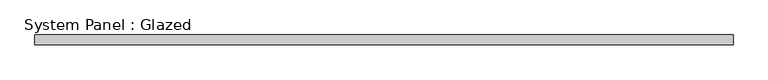
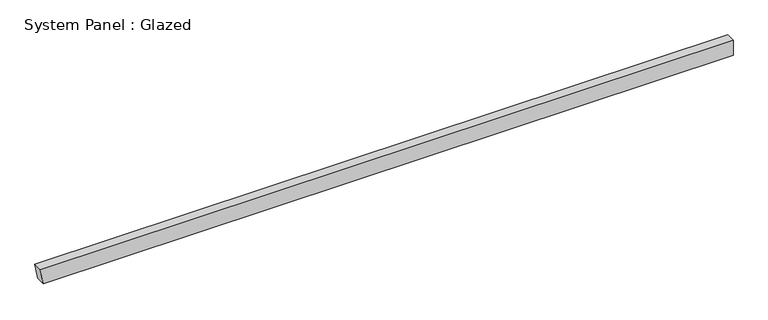
"""IFC4 building model written with IfcOpenShell, lengths in millimetres: plate geometry, System Panel : Glazed."""

from ifc_helpers import new_model, si_unit, frame, origin, place, context, project, spatial, polyline, outline, extrude, source, transform, mapped, element, save


def system_panel_glazed_0a43eb3e(model_context):
    return source(origin(), model_context, "Body", "SweptSolid", [
        extrude(outline(polyline([(0.0, -907.0374994), (0.0, 914.4000002), (41.9143134, 914.4000002), (41.9143134, -914.4000002), (0.0, -907.0374994)])), frame((0.0, -44.45, 0.0), z_axis=(0.0, 1.0, 0.0), x_axis=(0.0, 0.0, 1.0)), (0.0, 0.0, 1.0), 25.4),
    ])


if __name__ == "__main__":
    model = new_model("IFC4")
    model_context = context("Model", 3, world=origin())
    ifc_project = project(units=[si_unit("LENGTHUNIT", "METRE", prefix="MILLI")], contexts=[model_context])
    site = spatial("IfcSite", under=ifc_project)
    building = spatial("IfcBuilding", under=site)
    placement = place(None, origin())
    system_panel_glazed_shape = system_panel_glazed_0a43eb3e(model_context)
    element("IfcPlate", 1, ObjectType="System Panel : Glazed", at=placement, inside=building, context=model_context, shape_type="MappedRepresentation", body=[
        mapped(system_panel_glazed_shape, transform((0.0, 0.0, 0.0), x_axis=(1.0, 0.0, 0.0), y_axis=(0.0, 1.0, 0.0), z_axis=(0.0, 0.0, 1.0))),
    ])
    save(model, "model.ifc")

# Revit data of these elements
# Type "System Panel : Glazed"
#   Construction Type Id = "GSP4R"
#   Analytic Construction = "1/8 in Pilkington single glazing"
#   Visual Light Transmittance = 0.9
#   Solar Heat Gain Coefficient = 0.86
#   Heat Transfer Coefficient (U) = 1.18115 BTU/(h·ft²·°F)
#   Define Thermal Properties by = 1
# Element 1 (IfcPlate, "System Panel : Glazed")
#   Materials on its faces: "Glass"
# Materials
#   "Glass": class "Glass", colour RGB 0 128 192, transparency 0.75, Description = "Soda Lime Glass", Cost = 0
